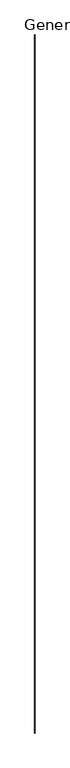
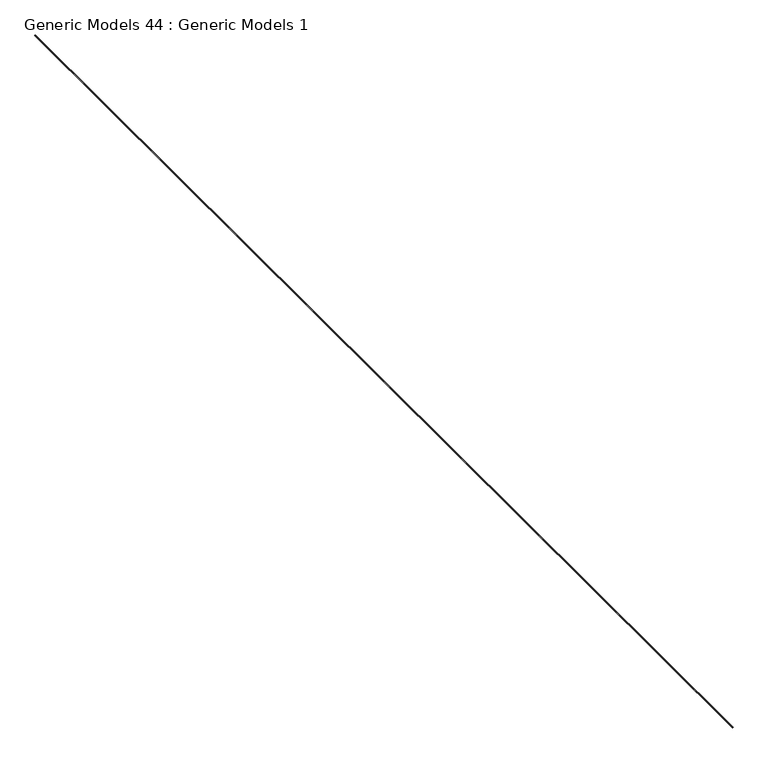
"""IFC4 building model written with IfcOpenShell, lengths in millimetres: proxy geometry, Generic Models 44 : Generic Models 1."""

from ifc_helpers import new_model, si_unit, point, frame, origin, place, context, project, spatial, polyline, circle_curve, ellipse_curve, trimmed, source, transform, mapped, element, save
from ifc_brep_helpers import plane_surface, cylinder_surface, revolved_surface, extruded_surface, advanced_brep


def generic_models_44_generic_models_1_7e2c46eb(model_context):
    return source(origin(), model_context, "Body", "AdvancedBrep", [
        advanced_brep(
        [(32090.3590778, 25672.1156612, 268881.225), (32090.3590778, 25672.1156612, 268874.875), (32093.5340778, 25672.1156612, 268874.875), (32094.4858371, 25672.1156612, 268876.1456586), (32094.4858371, 25672.1156612, 268879.9543414), (32093.5340778, 25672.1156612, 268881.225), (32090.3590778, 40827.6606612, 268881.225), (32093.5340778, 40827.6606612, 268881.225), (32094.4858371, 40827.6606612, 268879.9543414), (32094.4858371, 40827.6606612, 268876.1456586), (32093.5340778, 40827.6606612, 268874.875), (32090.3590778, 40827.6606612, 268874.875)],
        [
            (0, 1, circle_curve(frame((32087.4443373, 25672.1156612, 268878.05), z_axis=(0.0, 1.0, 0.0), x_axis=(0.0, 0.0, 1.0)), 4.3100275)),
            (1, 2),
            (2, 3, circle_curve(frame((32090.6193373, 25672.1156612, 268878.05), z_axis=(0.0, -1.0, 0.0), x_axis=(0.0, 0.0, 1.0)), 4.3100275)),
            (3, 4, ellipse_curve(frame((32098.2965778, 25672.1156612, 268878.05), z_axis=(0.0, -1.0, 0.0), x_axis=(-1.0, 0.0, 0.0)), 4.7625, 3.175)),
            (4, 5, circle_curve(frame((32090.6193373, 25672.1156612, 268878.05), z_axis=(0.0, -1.0, 0.0), x_axis=(0.0, 0.0, 1.0)), 4.3100275)),
            (5, 0),
            (6, 7),
            (7, 8, circle_curve(frame((32090.6193373, 40827.6606612, 268878.05), z_axis=(0.0, 1.0, 0.0), x_axis=(0.0, 0.0, 1.0)), 4.3100275)),
            (8, 9, ellipse_curve(frame((32098.2965778, 40827.6606612, 268878.05), z_axis=(0.0, 1.0, 0.0), x_axis=(-1.0, 0.0, 0.0)), 4.7625, 3.175)),
            (9, 10, circle_curve(frame((32090.6193373, 40827.6606612, 268878.05), z_axis=(0.0, 1.0, 0.0), x_axis=(0.0, 0.0, 1.0)), 4.3100275)),
            (10, 11),
            (11, 6, circle_curve(frame((32087.4443373, 40827.6606612, 268878.05), z_axis=(0.0, -1.0, 0.0), x_axis=(0.0, 0.0, 1.0)), 4.3100275)),
            (0, 6),
            (11, 1),
            (5, 7),
            (2, 10),
            (9, 3),
            (8, 4),
        ],
        [
            plane_surface(frame((32090.3590778, 25672.1156612, 268874.875), z_axis=(0.0, -1.0, 0.0), x_axis=(0.0, 0.0, 1.0))),
            plane_surface(frame((32090.3590778, 40827.6606612, 268874.875), z_axis=(0.0, 1.0, 0.0), x_axis=(0.0, 0.0, 1.0))),
            revolved_surface(polyline([(32087.4443373, 40827.6606612, 268882.36002749996), (32087.4443373, 25672.1156612, 268882.36002749996)]), (32087.4443373, 25672.1156612, 268878.05), (0.0, 1.0, 0.0)),
            plane_surface(frame((32093.5340778, 25672.1156612, 268881.225), z_axis=(0.0, 0.0, 1.0), x_axis=(0.0, 1.0, 0.0))),
            cylinder_surface(frame((32090.6193373, 25672.1156612, 268878.05), z_axis=(0.0, -1.0, 0.0), x_axis=(0.0, 0.0, 1.0)), 4.3100275),
            plane_surface(frame((32090.3590778, 25672.1156612, 268874.875), z_axis=(0.0, 0.0, -1.0), x_axis=(0.0, 1.0, 0.0))),
            extruded_surface(trimmed(ellipse_curve(frame((32098.2965778, 40827.6606612, 268878.05), z_axis=(0.0, -1.0, 0.0), x_axis=(-1.0, 0.0, 0.0)), 4.7625, 3.175), [point((32094.4858371, 40827.6606612, 268876.1456586))], [point((32094.4858371, 40827.6606612, 268879.9543414))], True, "CARTESIAN"), (0.0, -15155.545000000002, 0.0), 15155.545000000002),
        ],
        [
            (0, [[1, 2, 3, 4, 5, 6]]),
            (1, [[7, 8, 9, 10, 11, 12]]),
            (2, [[-1, 13, -12, 14]]),
            (3, [[-6, 15, -7, -13]]),
            (4, [[-3, 16, -10, 17]]),
            (5, [[-2, -14, -11, -16]]),
            (6, [[-4, -17, -9, 18]]),
            (4, [[-5, -18, -8, -15]]),
        ],
    ),
    ])


if __name__ == "__main__":
    model = new_model("IFC4")
    model_context = context("Model", 3, world=origin())
    ifc_project = project(units=[si_unit("LENGTHUNIT", "METRE", prefix="MILLI")], contexts=[model_context])
    site = spatial("IfcSite", under=ifc_project)
    building = spatial("IfcBuilding", under=site)
    placement = place(None, origin())
    generic_models_44_generic_models_1_shape = generic_models_44_generic_models_1_7e2c46eb(model_context)
    element("IfcBuildingElementProxy", 1, Name="Generic Models 44 : Generic Models 1", ObjectType="Generic Models 44 : Generic Models 1", at=placement, inside=building, context=model_context, shape_type="MappedRepresentation", body=[
        mapped(generic_models_44_generic_models_1_shape, transform((0.0, 0.0, 0.0), x_axis=(1.0, 0.0, 0.0), y_axis=(0.0, 1.0, 0.0), z_axis=(0.0, 0.0, 1.0))),
    ])
    save(model, "model.ifc")

# Revit data of these elements
# Element 1 (IfcBuildingElementProxy, "Generic Models 44 : Generic Models 1")
#   Materials on its faces: "SEALANT (& BACKER ROD IF NECESSARY)"
# Materials
#   "SEALANT (& BACKER ROD IF NECESSARY)": class "Generic", colour RGB 176 213 108, transparency 0, Cost = 0
